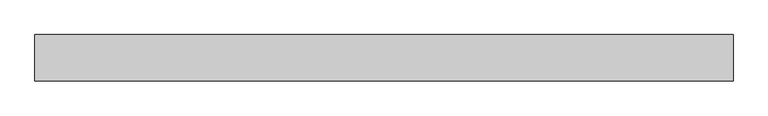
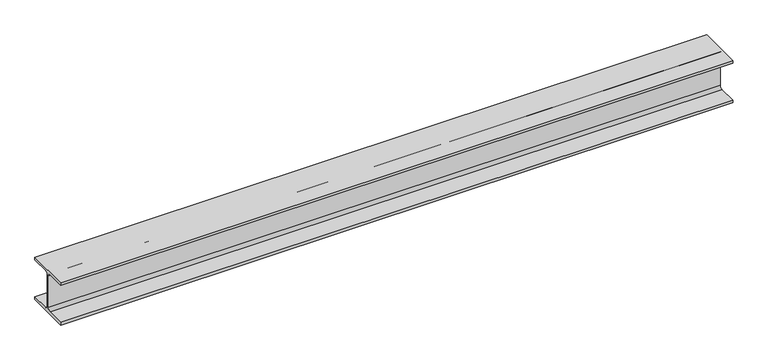
"""IFC4 building model written with IfcOpenShell, lengths in millimetres: beam geometry, 0912_Steel Framing_H-KSD3502 : H_SB_ASB_H-200x200x8x12."""

from ifc_helpers import new_model, si_unit, point, frame, frame_2d, origin, place, context, project, spatial, polyline, circle_curve, trimmed, segment, composite_curve, outline, extrude, source, transform, mapped, element, save


def beam_d9f12d6c(model_context):
    return source(origin(), model_context, "Body", "SweptSolid", [
        extrude(outline(composite_curve([segment(polyline([(100.0, -88.0), (100.0, -100.0), (-100.0, -100.0), (-100.0, -88.0), (-17.0, -88.0)]), True, "CONTINUOUS"), segment(trimmed(circle_curve(frame_2d((-17.0, -75.0)), 13.0), [point((-17.0, -88.0))], [point((-4.0, -75.0))], True, "CARTESIAN"), True, "CONTINUOUS"), segment(polyline([(-4.0, -75.0), (-4.0, 75.0)]), True, "CONTINUOUS"), segment(trimmed(circle_curve(frame_2d((-17.0, 75.0)), 13.0), [point((-4.0, 75.0))], [point((-17.0, 88.0))], True, "CARTESIAN"), True, "CONTINUOUS"), segment(polyline([(-17.0, 88.0), (-100.0, 88.0), (-100.0, 100.0), (100.0, 100.0), (100.0, 88.0), (17.0, 88.0)]), True, "CONTINUOUS"), segment(trimmed(circle_curve(frame_2d((17.0, 75.0)), 13.0), [point((17.0, 88.0))], [point((4.0, 75.0))], True, "CARTESIAN"), True, "CONTINUOUS"), segment(polyline([(4.0, 75.0), (4.0, -75.0)]), True, "CONTINUOUS"), segment(trimmed(circle_curve(frame_2d((17.0, -75.0)), 13.0), [point((4.0, -75.0))], [point((17.0, -88.0))], True, "CARTESIAN"), True, "CONTINUOUS"), segment(polyline([(17.0, -88.0), (100.0, -88.0)]), True, "CONTINUOUS")], self_intersect=False)), frame((-1314.165413, 0.0, 0.0), z_axis=(1.0, 0.0, 0.0), x_axis=(0.0, 1.0, 0.0)), (0.0, 0.0, 1.0), 3007.1539557),
    ])


if __name__ == "__main__":
    model = new_model("IFC4")
    model_context = context("Model", 3, world=origin())
    ifc_project = project(units=[si_unit("LENGTHUNIT", "METRE", prefix="MILLI")], contexts=[model_context])
    site = spatial("IfcSite", under=ifc_project)
    building = spatial("IfcBuilding", under=site)
    placement = place(None, origin())
    beam_shape = beam_d9f12d6c(model_context)
    element("IfcBeam", 1, ObjectType="0912_Steel Framing_H-KSD3502 : H_SB_ASB_H-200x200x8x12", at=placement, inside=building, context=model_context, shape_type="MappedRepresentation", body=[
        mapped(beam_shape, transform((0.0, 0.0, 0.0), x_axis=(1.0, 0.0, 0.0), y_axis=(0.0, 1.0, 0.0), z_axis=(0.0, 0.0, 1.0))),
    ])
    save(model, "model.ifc")

# Revit data of these elements
# Type "0912_Steel Framing_H-KSD3502 : H_SB_ASB_H-200x200x8x12"
#   H_WM Code_1 = "S01AA002-00001 | Main Steel Structure Fabrication Work | Shelter/Building | Medium Steel - Standard (90KG/M>Weight≥30KG/M) | Material: (   )"
#   H_WM Code_2 = "S03AA028-00001 | Main Steel Structure Erection Work | Shelter/Building | Medium Steel (90KG/M>Weight≥30KG/M) | Material: (   )"
#   H_WM Code_3 = "S01AA010-00001 | Main Steel Structure Fabrication Work | Shelter/Building | Steel Painting/Coating | for Non-Fireproofed Steel Surface, Surface Preparation, Primer, Second & Final Coat | Material: (   )"
#   H_Q'ty Cal Type Tag = "SB-Q2"
#   Width = 20.0 cm
#   Web Thickness = 0.8 cm
#   Web Fillet = 1.3 cm
#   Warping Constant = 141000.0 cm⁶
#   W = 0
#   Torsional Moment of Inertia = 26.2485 cm⁴
#   Section Area = 63.53 cm²
#   Plastic Modulus weak axis = 244.0 cm³
#   Plastic Modulus strong axis = 525.0 cm³
#   Perimeter = 1.16 m²/m
#   Nominal Weight = 49.90 kgf/m
#   Moment of Inertia weak axis = 1600.00 cm⁴
#   Moment of Inertia strong axis = 4720.00 cm⁴
#   Height = 20.0 cm
#   Flange Thickness = 1.2 cm
#   Elastic Modulus weak axis = 160.0 cm³
#   Elastic Modulus strong axis = 472.0 cm³
#   Centroid Vertical = 10.0 cm
#   Centroid Horizontal = 10.0 cm
#   Ix = 47200000
#   Length [instance default] = 1.5240 m
#   Zx = 525000
#   b = 0.2000 m
#   h = 0.2000 m
#   r = 0.0130 m
#   s = 0.0080 m
#   t = 0.0120 m
#   A = 0.006353 m²
#   Structural Material [instance default] = Steel, 45-345
#   Assembly Code = ""
# Element 1 (IfcBeam, "0912_Steel Framing_H-KSD3502 : H_SB_ASB_H-200x200x8x12")
#   Structural Material = none
# Materials
#   "Steel, 45-345": class "Metal", colour RGB 189 187 185, transparency 0, Description = "Steel 345 MPa", Cost = 0
